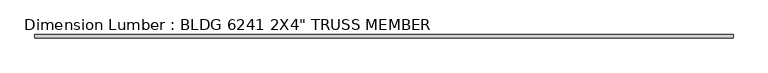
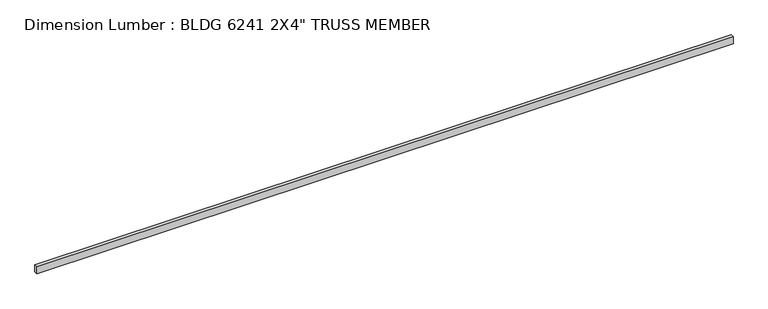
"""IFC4 building model written with IfcOpenShell, lengths in millimetres: beam geometry."""

from ifc_helpers import new_model, si_unit, frame, origin, place, context, project, spatial, polyline, outline, extrude, source, transform, mapped, element, save


def beam_8dd97a7c(model_context):
    return source(origin(), model_context, "Body", "SweptSolid", [
        extrude(outline(polyline([(5029.1999994, 25.4), (5029.1999994, -25.4), (-5029.1999994, -25.4), (-5029.1999994, 25.4), (5029.1999994, 25.4)])), frame((0.0, 0.0, -50.8), z_axis=(0.0, 0.0, 1.0), x_axis=(1.0, 0.0, 0.0)), (0.0, 0.0, 1.0), 101.6),
    ])


if __name__ == "__main__":
    model = new_model("IFC4")
    model_context = context("Model", 3, world=origin())
    ifc_project = project(units=[si_unit("LENGTHUNIT", "METRE", prefix="MILLI")], contexts=[model_context])
    site = spatial("IfcSite", under=ifc_project)
    building = spatial("IfcBuilding", under=site)
    placement = place(None, origin())
    beam_shape = beam_8dd97a7c(model_context)
    element("IfcBeam", 1, ObjectType="Dimension Lumber : BLDG 6241 2X4\" TRUSS MEMBER", at=placement, inside=building, context=model_context, shape_type="MappedRepresentation", body=[
        mapped(beam_shape, transform((0.0, 0.0, 0.0), x_axis=(1.0, 0.0, 0.0), y_axis=(0.0, 1.0, 0.0), z_axis=(0.0, 0.0, 1.0))),
    ])
    save(model, "model.ifc")

# Revit data of these elements
# Type "Dimension Lumber : BLDG 6241 2X4\" TRUSS MEMBER"
#   Assembly Code = "B10"
#   A = 0.273472 SF
#   Length [instance default] = 5' - 0"
#   b = 0' - 2"
#   d = 0' - 4"
#   Structural Material [instance default] = Softwood, Lumber
# Element 1 (IfcBeam, "Dimension Lumber : BLDG 6241 2X4\" TRUSS MEMBER")
#   Materials on its faces: "Softwood, Lumber"
# Materials
#   "Softwood, Lumber": class "Wood", colour RGB 223 192 134, transparency 0, Description = "Pinus Echinata", Cost = 0
